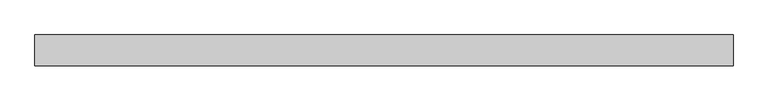
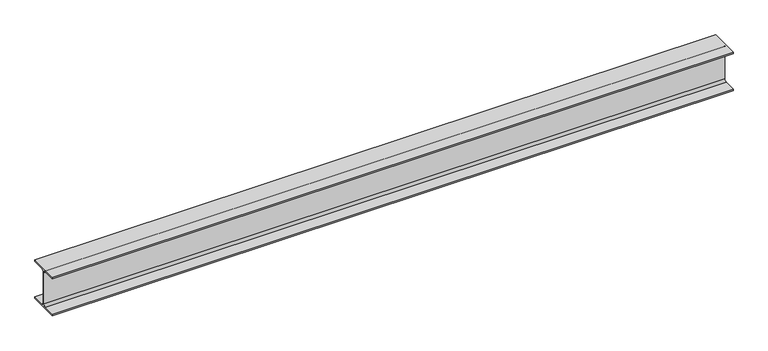
"""IFC4 building model written with IfcOpenShell, lengths in millimetres: beam geometry, 0912_Steel Framing_H-KSD3502 : H_SB_ASB_H-340x250x9x14."""

import ifcopenshell
import ifcopenshell.guid

model = None  # the IFC model being written
_history = None  # IfcOwnerHistory: only IFC2X3 demands one
_inside = {}  # id of a spatial element -> (the spatial element, [elements in it])
_under = {}  # id of a project, library or spatial element -> (it, [spatial elements below it])
_declared = {}  # id of a project -> (the project, [libraries it declares])
_typed = {}  # id of a type object -> (the type object, [elements of that type])
_made_of = {}  # id of a material, layer set ... -> (it, [elements and type objects made of it])


def new_model(schema):
    """Start an empty IFC model of exactly this schema.

    Asked for "IFC4X3", IfcOpenShell would pick the latest addendum, in which some entities
    have other attributes; the version numbers below select the first issue.
    IFC2X3 requires an IfcOwnerHistory on every rooted entity: one is made here for all.
    """
    global model, _history
    if schema == "IFC4X3":
        model = ifcopenshell.file(schema_version=(4, 3, 0, 0))
    else:
        model = ifcopenshell.file(schema=schema)
    _inside.clear()
    _under.clear()
    _declared.clear()
    _typed.clear()
    _made_of.clear()
    _history = None
    if model.schema == "IFC2X3":
        org = make("IfcOrganization", Name="unknown")
        user = make(
            "IfcPersonAndOrganization",
            ThePerson=make("IfcPerson", FamilyName="unknown"),
            TheOrganization=org,
        )
        app = make(
            "IfcApplication",
            ApplicationDeveloper=org,
            Version="unknown",
            ApplicationFullName="unknown",
            ApplicationIdentifier="unknown",
        )
        _history = make(
            "IfcOwnerHistory",
            OwningUser=user,
            OwningApplication=app,
            ChangeAction="ADDED",
            CreationDate=0,
        )
    return model


def make(cls, **values):
    """One entity of the class cls with the attributes given. An attribute that is None is left unset."""
    return model.create_entity(
        cls, **{name: value for name, value in values.items() if value is not None}
    )


def rooted(cls, **values):
    """An entity with a GlobalId (a new one), such as an element, a storey or a relation."""
    return make(cls, GlobalId=ifcopenshell.guid.new(), OwnerHistory=_history, **values)


def si_unit(unit_type, name, prefix=None):
    """IfcSIUnit, for example si_unit("LENGTHUNIT", "METRE", prefix="MILLI")."""
    return make("IfcSIUnit", UnitType=unit_type, Prefix=prefix, Name=name)


def assignment(units):
    """IfcUnitAssignment: the units of a project."""
    return None if units is None else make("IfcUnitAssignment", Units=units)


def point(xyz):
    """IfcCartesianPoint."""
    return None if xyz is None else make("IfcCartesianPoint", Coordinates=xyz)


def direction(xyz):
    """IfcDirection."""
    return None if xyz is None else make("IfcDirection", DirectionRatios=xyz)


def frame(location, z_axis=None, x_axis=None):
    """IfcAxis2Placement3D, a coordinate frame: its origin and axes. An axis left out is left unset."""
    return make(
        "IfcAxis2Placement3D",
        Location=point(location),
        Axis=direction(z_axis),
        RefDirection=direction(x_axis),
    )


def frame_2d(location, x_axis=None):
    """IfcAxis2Placement2D, a coordinate frame in the plane: its origin and x axis."""
    return make(
        "IfcAxis2Placement2D", Location=point(location), RefDirection=direction(x_axis)
    )


def origin():
    """The frame at (0, 0, 0) with its axes left unset."""
    return frame((0.0, 0.0, 0.0))


def place(relative_to, where):
    """IfcLocalPlacement: puts the frame where relative to a parent placement (None: the world)."""
    return make(
        "IfcLocalPlacement", PlacementRelTo=relative_to, RelativePlacement=where
    )


def context(
    kind, dimensions, precision=None, world=None, true_north=None, identifier=None
):
    """IfcGeometricRepresentationContext, for example the 3D "Model" context."""
    return make(
        "IfcGeometricRepresentationContext",
        ContextIdentifier=identifier,
        ContextType=kind,
        CoordinateSpaceDimension=dimensions,
        Precision=precision,
        WorldCoordinateSystem=world,
        TrueNorth=true_north,
    )


def project(units=None, contexts=None):
    """IfcProject with its units and contexts."""
    return rooted(
        "IfcProject",
        Name="project",
        RepresentationContexts=contexts,
        UnitsInContext=assignment(units),
    )


def spatial(cls, under=None, at=None, **own):
    """A site, building, storey or space (cls), placed at a placement, below another one or the project."""
    s = rooted(cls, ObjectPlacement=at, **own)
    if under is not None:
        _under.setdefault(under.id(), (under, []))[1].append(s)
    return s


def polyline(points):
    """IfcPolyline through the points."""
    return make("IfcPolyline", Points=[point(p) for p in points])


def circle_curve(where, radius):
    """IfcCircle in the frame where."""
    return make("IfcCircle", Position=where, Radius=radius)


def trimmed(basis, trim1, trim2, sense, master):
    """IfcTrimmedCurve: the piece of a basis curve between two trims."""
    return make(
        "IfcTrimmedCurve",
        BasisCurve=basis,
        Trim1=trim1,
        Trim2=trim2,
        SenseAgreement=sense,
        MasterRepresentation=master,
    )


def segment(curve, same_sense, transition):
    """IfcCompositeCurveSegment."""
    return make(
        "IfcCompositeCurveSegment",
        Transition=transition,
        SameSense=same_sense,
        ParentCurve=curve,
    )


def composite_curve(segments, self_intersect=None):
    """IfcCompositeCurve: segments joined end to end."""
    return make("IfcCompositeCurve", Segments=segments, SelfIntersect=self_intersect)


def outline(outer, holes=None, kind="AREA"):
    """IfcArbitraryClosedProfileDef: a profile drawn as a closed curve; with holes, ...WithVoids."""
    if holes is None:
        return make("IfcArbitraryClosedProfileDef", ProfileType=kind, OuterCurve=outer)
    return make(
        "IfcArbitraryProfileDefWithVoids",
        ProfileType=kind,
        OuterCurve=outer,
        InnerCurves=holes,
    )


def extrude(swept, where, along, depth):
    """IfcExtrudedAreaSolid: the profile swept, set in the frame where, extruded along a direction by depth."""
    return make(
        "IfcExtrudedAreaSolid",
        SweptArea=swept,
        Position=where,
        ExtrudedDirection=direction(along),
        Depth=depth,
    )


def shape(context_of_items, identifier, shape_type, items):
    """IfcShapeRepresentation: the items that make up one representation, for example the "Body"."""
    return make(
        "IfcShapeRepresentation",
        ContextOfItems=context_of_items,
        RepresentationIdentifier=identifier,
        RepresentationType=shape_type,
        Items=items,
    )


def source(mapping_origin, context_of_items, identifier, shape_type, items):
    """IfcRepresentationMap: a shape defined once, which mapped items show again and again."""
    return make(
        "IfcRepresentationMap",
        MappingOrigin=mapping_origin,
        MappedRepresentation=shape(context_of_items, identifier, shape_type, items),
    )


def transform(
    local_origin,
    x_axis=None,
    y_axis=None,
    z_axis=None,
    scale=None,
    scale2=None,
    scale3=None,
    uniform=True,
):
    """IfcCartesianTransformationOperator3D, or its non-uniform kind. x_axis, y_axis, z_axis: its Axis1, 2, 3."""
    if uniform:
        return make(
            "IfcCartesianTransformationOperator3D",
            Axis1=direction(x_axis),
            Axis2=direction(y_axis),
            LocalOrigin=point(local_origin),
            Scale=scale,
            Axis3=direction(z_axis),
        )
    return make(
        "IfcCartesianTransformationOperator3DnonUniform",
        Axis1=direction(x_axis),
        Axis2=direction(y_axis),
        LocalOrigin=point(local_origin),
        Scale=scale,
        Axis3=direction(z_axis),
        Scale2=scale2,
        Scale3=scale3,
    )


def mapped(mapping_source, mapping_target):
    """IfcMappedItem: shows the shape of a source again, moved by a transform."""
    return make(
        "IfcMappedItem", MappingSource=mapping_source, MappingTarget=mapping_target
    )


def made_of(thing, what):
    """Note that an element or type object is made of a material, layer set ...; save() writes the relation."""
    if what is not None:
        _made_of.setdefault(what.id(), (what, []))[1].append(thing)
    return thing


def element(
    cls,
    number,
    at=None,
    inside=None,
    cuts=None,
    type_object=None,
    material=None,
    context=None,
    identifier="Body",
    shape_type=None,
    held_by="IfcProductDefinitionShape",
    body=None,
    shapes=None,
    **own,
):
    """One element of the class cls, such as IfcWall. Its Tag is "e" and its number.

    at: its placement. inside: the storey or other place that contains it. cuts: it is an
    opening in that element (IfcRelVoidsElement). A single representation is given by context,
    identifier, shape_type and body (its items); several are given by shapes. held_by: the class
    of the entity that holds the representations. save() writes the other relations.
    """
    e = rooted(cls, Tag="e%d" % number, ObjectPlacement=at, **own)
    if body is not None:
        shapes = [shape(context, identifier, shape_type, body)]
    if shapes is not None:
        e.Representation = make(held_by, Representations=shapes)
    if inside is not None:
        _inside.setdefault(inside.id(), (inside, []))[1].append(e)
    if cuts is not None:
        rooted(
            "IfcRelVoidsElement", RelatingBuildingElement=cuts, RelatedOpeningElement=e
        )
    if type_object is not None:
        _typed.setdefault(type_object.id(), (type_object, []))[1].append(e)
    return made_of(e, material)


def aggregate(whole, parts):
    """IfcRelAggregates: a whole, such as a stair, and the parts it consists of."""
    return rooted("IfcRelAggregates", RelatingObject=whole, RelatedObjects=parts)


def save(model, path):
    """Write the relations noted so far, then the file.

    IfcRelAggregates (storeys below a building ...), IfcRelContainedInSpatialStructure (elements
    in a storey), IfcRelDefinesByType, IfcRelAssociatesMaterial and IfcRelDeclares: one each for
    every whole, place, type object, material and project.
    """
    for whole, parts in _under.values():
        aggregate(whole, parts)
    for where, things in _inside.values():
        rooted(
            "IfcRelContainedInSpatialStructure",
            RelatedElements=things,
            RelatingStructure=where,
        )
    for kind, things in _typed.values():
        rooted("IfcRelDefinesByType", RelatedObjects=things, RelatingType=kind)
    for what, things in _made_of.values():
        rooted("IfcRelAssociatesMaterial", RelatedObjects=things, RelatingMaterial=what)
    for by, libraries in _declared.values():
        rooted("IfcRelDeclares", RelatingContext=by, RelatedDefinitions=libraries)
    model.write(path)


def beam_b7f7b6e9(model_context):
    return source(origin(), model_context, "Body", "SweptSolid", [
        extrude(outline(composite_curve([segment(polyline([(125.0, -156.0), (125.0, -170.0), (-125.0, -170.0), (-125.0, -156.0), (-24.5, -156.0)]), True, "CONTINUOUS"), segment(trimmed(circle_curve(frame_2d((-24.5, -136.0)), 20.0), [point((-24.5, -156.0))], [point((-4.5, -136.0))], True, "CARTESIAN"), True, "CONTINUOUS"), segment(polyline([(-4.5, -136.0), (-4.5, 136.0)]), True, "CONTINUOUS"), segment(trimmed(circle_curve(frame_2d((-24.5, 136.0)), 20.0), [point((-4.5, 136.0))], [point((-24.5, 156.0))], True, "CARTESIAN"), True, "CONTINUOUS"), segment(polyline([(-24.5, 156.0), (-125.0, 156.0), (-125.0, 170.0), (125.0, 170.0), (125.0, 156.0), (24.5, 156.0)]), True, "CONTINUOUS"), segment(trimmed(circle_curve(frame_2d((24.5, 136.0)), 20.0), [point((24.5, 156.0))], [point((4.5, 136.0))], True, "CARTESIAN"), True, "CONTINUOUS"), segment(polyline([(4.5, 136.0), (4.5, -136.0)]), True, "CONTINUOUS"), segment(trimmed(circle_curve(frame_2d((24.5, -136.0)), 20.0), [point((4.5, -136.0))], [point((24.5, -156.0))], True, "CARTESIAN"), True, "CONTINUOUS"), segment(polyline([(24.5, -156.0), (125.0, -156.0)]), True, "CONTINUOUS")], self_intersect=False)), frame((-2837.3, 0.0, 0.0), z_axis=(1.0, 0.0, 0.0), x_axis=(0.0, 1.0, 0.0)), (0.0, 0.0, 1.0), 5674.6),
    ])


if __name__ == "__main__":
    model = new_model("IFC4")
    model_context = context("Model", 3, world=origin())
    ifc_project = project(units=[si_unit("LENGTHUNIT", "METRE", prefix="MILLI")], contexts=[model_context])
    site = spatial("IfcSite", under=ifc_project)
    building = spatial("IfcBuilding", under=site)
    placement = place(None, origin())
    beam_shape = beam_b7f7b6e9(model_context)
    element("IfcBeam", 1, ObjectType="0912_Steel Framing_H-KSD3502 : H_SB_ASB_H-340x250x9x14", at=placement, inside=building, context=model_context, shape_type="MappedRepresentation", body=[
        mapped(beam_shape, transform((0.0, 0.0, 0.0), x_axis=(1.0, 0.0, 0.0), y_axis=(0.0, 1.0, 0.0), z_axis=(0.0, 0.0, 1.0))),
    ])
    save(model, "model.ifc")

# Revit data of these elements
# Type "0912_Steel Framing_H-KSD3502 : H_SB_ASB_H-340x250x9x14"
#   H_WM Code_1 = "S01AA002-00001 | Main Steel Structure Fabrication Work | Shelter/Building | Medium Steel - Standard (90KG/M>Weight≥30KG/M) | Material: (   )"
#   H_WM Code_2 = "S03AA028-00001 | Main Steel Structure Erection Work | Shelter/Building | Medium Steel (90KG/M>Weight≥30KG/M) | Material: (   )"
#   H_WM Code_3 = "S01AA010-00001 | Main Steel Structure Fabrication Work | Shelter/Building | Steel Painting/Coating | for Non-Fireproofed Steel Surface, Surface Preparation, Primer, Second & Final Coat | Material: (   )"
#   H_Q'ty Cal Type Tag = "SB-Q2"
#   Width = 25.0 cm
#   Web Thickness = 0.9 cm
#   Web Fillet = 2.0 cm
#   Warping Constant = 969000.0 cm⁶
#   W = 0
#   Torsional Moment of Inertia = 53.6551 cm⁴
#   Section Area = 101.5 cm²
#   Plastic Modulus weak axis = 447.0 cm³
#   Plastic Modulus strong axis = 1410.0 cm³
#   Perimeter = 1.63 m²/m
#   Nominal Weight = 79.70 kgf/m
#   Moment of Inertia weak axis = 3650.00 cm⁴
#   Moment of Inertia strong axis = 21700.00 cm⁴
#   Height = 34.0 cm
#   Flange Thickness = 1.4 cm
#   Elastic Modulus weak axis = 292.0 cm³
#   Elastic Modulus strong axis = 1280.0 cm³
#   Centroid Vertical = 17.0 cm
#   Centroid Horizontal = 12.5 cm
#   Ix = 217000000
#   Length [instance default] = 1.5240 m
#   Zx = 1410000
#   b = 0.2500 m
#   h = 0.3400 m
#   r = 0.0200 m
#   s = 0.0090 m
#   t = 0.0140 m
#   A = 0.01015 m²
#   Structural Material [instance default] = Steel, 45-345
#   Assembly Code = ""
# Element 1 (IfcBeam, "0912_Steel Framing_H-KSD3502 : H_SB_ASB_H-340x250x9x14")
#   Structural Material = none
# Materials
#   "Steel, 45-345": class "Metal", colour RGB 189 187 185, transparency 0, Description = "Steel 345 MPa", Cost = 0
